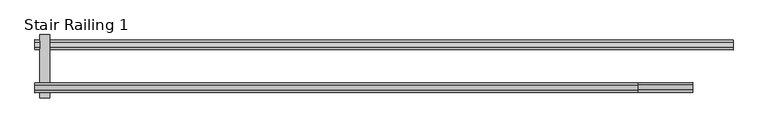
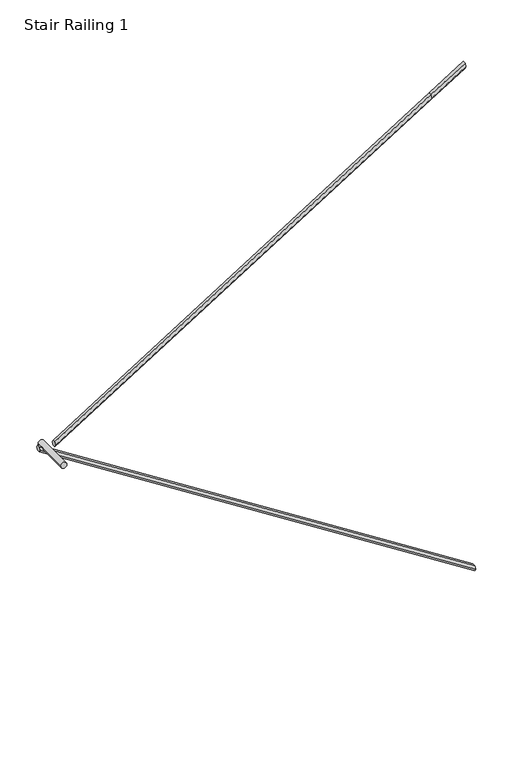
"""IFC4 building model written with IfcOpenShell, lengths in millimetres: railing geometry, Stair Railing 1."""

from ifc_helpers import new_model, si_unit, frame, origin, place, context, project, spatial, circle_curve, faceted_brep, source, transform, mapped, element, save
from ifc_brep_helpers import plane_surface, cylinder_surface, advanced_brep


def stair_railing_1_ea28da98(model_context):
    return source(origin(), model_context, "Body", "SolidModel", [
        faceted_brep([(46974.7398084, 46191.4865351, 9028.2888889), (46974.7398084, 46204.1865351, 9050.2859341), (46974.7398084, 46229.5865351, 9050.2859341), (46974.7398084, 46242.2865351, 9028.2888889), (46974.7398084, 46229.5865351, 9006.2918436), (46974.7398084, 46204.1865351, 9006.2918436), (50533.2139908, 46191.4865351, 6753.5777778), (50533.2139908, 46204.1865351, 6731.5807325), (50533.2139908, 46229.5865351, 6731.5807325), (50533.2139908, 46242.2865351, 6753.5777778), (50533.2139908, 46229.5865351, 6775.574823), (50533.2139908, 46204.1865351, 6775.574823)], [[[0, 1, 2, 3, 4, 5]], [[6, 7, 8, 9, 10, 11]], [[1, 0, 6, 11]], [[2, 1, 11, 10]], [[3, 2, 10, 9]], [[4, 3, 9, 8]], [[5, 4, 8, 7]], [[0, 5, 7, 6]]]),
        advanced_brep(
        [(47050.9398084, 45946.4030566, 9028.2888889), (47000.1398084, 45946.4030566, 9028.2888889), (47050.9398084, 46267.6865351, 9028.2888889), (47000.1398084, 46267.6865351, 9028.2888889)],
        [
            (0, 1, circle_curve(frame((47025.5398084, 45946.4030566, 9028.2888889), z_axis=(0.0, -1.0, 0.0), x_axis=(1.0, 0.0, 0.0)), 25.4)),
            (1, 0, circle_curve(frame((47025.5398084, 45946.4030566, 9028.2888889), z_axis=(0.0, -1.0, 0.0), x_axis=(1.0, 0.0, 0.0)), 25.4)),
            (2, 3, circle_curve(frame((47025.5398084, 46267.6865351, 9028.2888889), z_axis=(0.0, 1.0, 0.0), x_axis=(1.0, 0.0, 0.0)), 25.4)),
            (3, 2, circle_curve(frame((47025.5398084, 46267.6865351, 9028.2888889), z_axis=(0.0, 1.0, 0.0), x_axis=(1.0, 0.0, 0.0)), 25.4)),
            (0, 2),
            (3, 1),
        ],
        [
            plane_surface(frame((47050.9398084, 45946.4030566, 9002.8888889), z_axis=(0.0, -1.0, 0.0), x_axis=(0.0, 0.0, -1.0))),
            plane_surface(frame((47050.9398084, 46267.6865351, 9002.8888889), z_axis=(0.0, 1.0, 0.0), x_axis=(0.0, 0.0, 1.0))),
            cylinder_surface(frame((47025.5398084, 46267.6865351, 9028.2888889), z_axis=(0.0, -1.0, 0.0), x_axis=(1.0, 0.0, 0.0)), 25.4),
        ],
        [
            (0, [[1, 2]]),
            (1, [[3, 4]]),
            (2, [[-1, 5, -4, 6]]),
            (2, [[-2, -6, -3, -5]]),
        ],
    ),
        faceted_brep([(50048.1398084, 46022.6030566, 11128.0222222), (50048.1398084, 46009.9030566, 11150.0192675), (50048.1398084, 45984.5030566, 11150.0192675), (50048.1398084, 45971.8030566, 11128.0222222), (50048.1398084, 45984.5030566, 11106.025177), (50048.1398084, 46009.9030566, 11106.025177), (46974.7398084, 46022.6030566, 9203.2666667), (46974.7398084, 46009.9030566, 9181.2696214), (46974.7398084, 45984.5030566, 9181.2696214), (46974.7398084, 45971.8030566, 9203.2666667), (46974.7398084, 45984.5030566, 9225.2637119), (46974.7398084, 46009.9030566, 9225.2637119)], [[[0, 1, 2, 3, 4, 5]], [[6, 7, 8, 9, 10, 11]], [[1, 0, 6, 11]], [[2, 1, 11, 10]], [[3, 2, 10, 9]], [[4, 3, 9, 8]], [[5, 4, 8, 7]], [[0, 5, 7, 6]]]),
        faceted_brep([(50327.5398084, 46022.6030566, 11303.0), (50327.5398084, 46009.9030566, 11324.9970453), (50327.5398084, 45984.5030566, 11324.9970453), (50327.5398084, 45971.8030566, 11303.0), (50327.5398084, 45984.5030566, 11281.0029547), (50327.5398084, 46009.9030566, 11281.0029547), (50048.1398084, 46022.6030566, 11128.0222222), (50048.1398084, 46009.9030566, 11106.025177), (50048.1398084, 45984.5030566, 11106.025177), (50048.1398084, 45971.8030566, 11128.0222222), (50048.1398084, 45984.5030566, 11150.0192675), (50048.1398084, 46009.9030566, 11150.0192675)], [[[0, 1, 2, 3, 4, 5]], [[6, 7, 8, 9, 10, 11]], [[1, 0, 6, 11]], [[2, 1, 11, 10]], [[3, 2, 10, 9]], [[4, 3, 9, 8]], [[5, 4, 8, 7]], [[0, 5, 7, 6]]]),
    ])


if __name__ == "__main__":
    model = new_model("IFC4")
    model_context = context("Model", 3, world=origin())
    ifc_project = project(units=[si_unit("LENGTHUNIT", "METRE", prefix="MILLI")], contexts=[model_context])
    site = spatial("IfcSite", under=ifc_project)
    building = spatial("IfcBuilding", under=site)
    placement = place(None, origin())
    stair_railing_1_shape = stair_railing_1_ea28da98(model_context)
    element("IfcRailing", 1, ObjectType="Stair Railing 1", at=placement, inside=building, context=model_context, shape_type="MappedRepresentation", body=[
        mapped(stair_railing_1_shape, transform((0.0, 0.0, 0.0), x_axis=(1.0, 0.0, 0.0), y_axis=(0.0, 1.0, 0.0), z_axis=(0.0, 0.0, 1.0))),
    ])
    save(model, "model.ifc")
